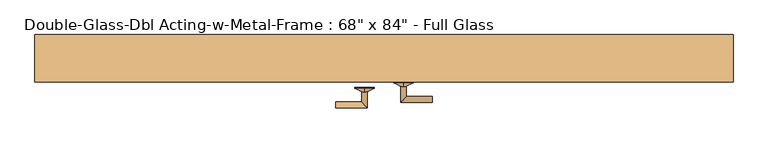
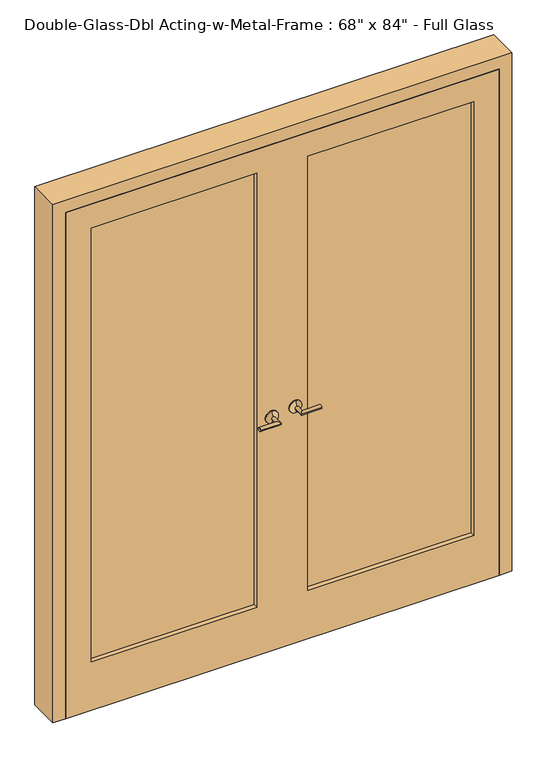
"""IFC4 building model written with IfcOpenShell, lengths in millimetres: door geometry."""

from ifc_helpers import new_model, si_unit, point, frame, origin, place, context, project, spatial, polyline, circle_curve, ellipse_curve, trimmed, outline, extrude, source, transform, mapped, element, save
from ifc_brep_helpers import plane_surface, cylinder_surface, revolved_surface, advanced_brep


def door_4d2e2016(model_context):
    return source(origin(), model_context, "Body", "SolidModel", [
        advanced_brep(
        [(50.8, -28.575, 971.55), (50.8, -28.575, 1022.35), (50.8, -20.0863821, 1004.45), (43.3, -20.0863821, 996.95), (50.8, -20.0863821, 989.45), (58.3, -20.0863821, 996.95), (50.8, -31.75, 971.55), (50.8, -31.75, 1022.35), (50.8, -31.75, 996.95), (43.3, 21.85, 996.95), (58.3, 6.85, 996.95), (125.8, 21.85, 996.95), (125.8, 6.85, 996.95)],
        [
            (0, 1, circle_curve(frame((50.8, -28.575, 996.95), z_axis=(0.0, 1.0, 0.0), x_axis=(0.0, 0.0, 1.0)), 25.4)),
            (1, 2, circle_curve(frame((50.8, 8.0292775, 1028.7458887), z_axis=(1.0000000000000004, 0.0, 0.0), x_axis=(0.0, 0.0, -1.0)), 37.1588553)),
            (2, 3, circle_curve(frame((50.8, -20.0863821, 996.95), z_axis=(0.0, -1.0, 0.0), x_axis=(0.0, 0.0, 1.0)), 7.5)),
            (3, 4, circle_curve(frame((50.8, -20.0863821, 996.95), z_axis=(0.0, -1.0, 0.0), x_axis=(0.0, 0.0, 1.0)), 7.5)),
            (4, 0, circle_curve(frame((50.8, 8.0292775, 965.1541113), z_axis=(1.0000000000000004, 0.0, 0.0), x_axis=(0.0, 0.0, 1.0)), 37.1588553)),
            (1, 0, circle_curve(frame((50.8, -28.575, 996.95), z_axis=(0.0, 1.0, 0.0), x_axis=(0.0, 0.0, 1.0)), 25.4)),
            (4, 5, circle_curve(frame((50.8, -20.0863821, 996.95), z_axis=(0.0, -1.0, 0.0), x_axis=(0.0, 0.0, 1.0)), 7.5)),
            (5, 2, circle_curve(frame((50.8, -20.0863821, 996.95), z_axis=(0.0, -1.0, 0.0), x_axis=(0.0, 0.0, 1.0)), 7.5)),
            (0, 6),
            (6, 7, circle_curve(frame((50.8, -31.75, 996.95), z_axis=(0.0, 1.0, 0.0), x_axis=(0.0, 0.0, 1.0)), 25.4)),
            (7, 1),
            (7, 6, circle_curve(frame((50.8, -31.75, 996.95), z_axis=(0.0, 1.0, 0.0), x_axis=(0.0, 0.0, 1.0)), 25.4)),
            (6, 8),
            (8, 7),
            (9, 10, ellipse_curve(frame((50.8, 14.35, 996.95), z_axis=(-0.7071067811864719, -0.7071067811866231, 0.0), x_axis=(0.707106781186623, -0.7071067811864721, 0.0)), 10.6066017, 7.5)),
            (10, 5),
            (3, 9),
            (10, 9, ellipse_curve(frame((50.8, 14.35, 996.95), z_axis=(-0.7071067811864719, -0.7071067811866231, 0.0), x_axis=(0.707106781186623, -0.7071067811864721, 0.0)), 10.6066017, 7.5)),
            (11, 12, circle_curve(frame((125.8, 14.35, 996.95), z_axis=(1.0, 0.0, 0.0), x_axis=(0.0, -1.0000000000000004, 0.0)), 7.5)),
            (12, 11, circle_curve(frame((125.8, 14.35, 996.95), z_axis=(1.0, 0.0, 0.0), x_axis=(0.0, -1.0000000000000004, 0.0)), 7.5)),
            (9, 11),
            (12, 10),
        ],
        [
            revolved_surface(trimmed(ellipse_curve(frame((50.8, 8.0292775, 1028.7458887), z_axis=(-1.0000000000000004, 0.0, 0.0), x_axis=(0.0, 0.0, -1.0)), 37.1588553, 37.1588553), [point((50.8, -19.05, 1003.3))], [point((50.8, -28.575, 1022.35))], True, "CARTESIAN"), (50.8, -19.05, 996.95), (0.0, -1.0000000000000004, 0.0)),
            cylinder_surface(frame((50.8, -19.05, 996.95), z_axis=(0.0, -1.0000000000000004, 0.0), x_axis=(0.0, 0.0, 1.0)), 25.4),
            plane_surface(frame((50.8, -31.75, 996.95), z_axis=(0.0, -1.0, 0.0), x_axis=(0.0, 0.0, 1.0))),
            cylinder_surface(frame((50.8, -23.75, 996.95), z_axis=(0.0, -1.0000000000000004, 0.0), x_axis=(1.0000000000000004, 0.0, 0.0)), 7.5),
            plane_surface(frame((125.8, 14.35, 996.95), z_axis=(1.0, 0.0, 0.0), x_axis=(0.0, 0.0, 1.0))),
            cylinder_surface(frame((50.8, 14.35, 996.95), z_axis=(-1.0000000000000004, 0.0, 0.0), x_axis=(0.0, -1.0000000000000004, 0.0)), 7.5),
        ],
        [
            (0, [[1, 2, 3, 4, 5]]),
            (0, [[6, -5, 7, 8, -2]]),
            (1, [[-1, 9, 10, 11]]),
            (1, [[-6, -11, 12, -9]]),
            (2, [[-10, 13, 14]]),
            (2, [[-12, -14, -13]]),
            (3, [[15, 16, -7, -4, 17]]),
            (3, [[18, -17, -3, -8, -16]]),
            (4, [[19, 20]]),
            (5, [[-15, 21, -20, 22]]),
            (5, [[-18, -22, -19, -21]]),
        ],
    ),
        advanced_brep(
        [(-50.8, -79.375, 971.55), (-50.8, -79.375, 1022.35), (-50.8, -87.8636179, 1004.45), (-43.3, -87.8636179, 996.95), (-50.8, -87.8636179, 989.45), (-58.3, -87.8636179, 996.95), (-50.8, -76.2, 971.55), (-50.8, -76.2, 1022.35), (-50.8, -76.2, 996.95), (-43.3, -129.8, 996.95), (-58.3, -114.8, 996.95), (-125.8, -129.8, 996.95), (-125.8, -114.8, 996.95)],
        [
            (0, 1, circle_curve(frame((-50.8, -79.375, 996.95), z_axis=(0.0, -1.0, 0.0), x_axis=(0.0, 0.0, 1.0)), 25.4)),
            (1, 2, circle_curve(frame((-50.8, -115.9792775, 1028.7458887), z_axis=(-1.0, 0.0, 0.0), x_axis=(0.0, 0.0, -1.0)), 37.1588553)),
            (2, 3, circle_curve(frame((-50.8, -87.8636179, 996.95), z_axis=(0.0, 1.0, 0.0), x_axis=(0.0, 0.0, 1.0)), 7.5)),
            (3, 4, circle_curve(frame((-50.8, -87.8636179, 996.95), z_axis=(0.0, 1.0, 0.0), x_axis=(0.0, 0.0, 1.0)), 7.5)),
            (4, 0, circle_curve(frame((-50.8, -115.9792775, 965.1541113), z_axis=(-1.0, 0.0, 0.0), x_axis=(0.0, 0.0, 1.0)), 37.1588553)),
            (1, 0, circle_curve(frame((-50.8, -79.375, 996.95), z_axis=(0.0, -1.0, 0.0), x_axis=(0.0, 0.0, 1.0)), 25.4)),
            (4, 5, circle_curve(frame((-50.8, -87.8636179, 996.95), z_axis=(0.0, 1.0, 0.0), x_axis=(0.0, 0.0, 1.0)), 7.5)),
            (5, 2, circle_curve(frame((-50.8, -87.8636179, 996.95), z_axis=(0.0, 1.0, 0.0), x_axis=(0.0, 0.0, 1.0)), 7.5)),
            (0, 6),
            (6, 7, circle_curve(frame((-50.8, -76.2, 996.95), z_axis=(0.0, -1.0, 0.0), x_axis=(0.0, 0.0, 1.0)), 25.4)),
            (7, 1),
            (7, 6, circle_curve(frame((-50.8, -76.2, 996.95), z_axis=(0.0, -1.0, 0.0), x_axis=(0.0, 0.0, 1.0)), 25.4)),
            (6, 8),
            (8, 7),
            (9, 10, ellipse_curve(frame((-50.8, -122.3, 996.95), z_axis=(0.7071067811864695, 0.7071067811866254, 0.0), x_axis=(-0.7071067811866254, 0.7071067811864696, 0.0)), 10.6066017, 7.5)),
            (10, 5),
            (3, 9),
            (10, 9, ellipse_curve(frame((-50.8, -122.3, 996.95), z_axis=(0.7071067811864695, 0.7071067811866254, 0.0), x_axis=(-0.7071067811866254, 0.7071067811864696, 0.0)), 10.6066017, 7.5)),
            (11, 12, circle_curve(frame((-125.8, -122.3, 996.95), z_axis=(-1.0, 0.0, 0.0), x_axis=(0.0, 1.0, 0.0)), 7.5)),
            (12, 11, circle_curve(frame((-125.8, -122.3, 996.95), z_axis=(-1.0, 0.0, 0.0), x_axis=(0.0, 1.0, 0.0)), 7.5)),
            (9, 11),
            (12, 10),
        ],
        [
            revolved_surface(trimmed(ellipse_curve(frame((-50.8, -115.9792775, 1028.7458887), z_axis=(1.0, 0.0, 0.0), x_axis=(0.0, 0.0, -1.0)), 37.1588553, 37.1588553), [point((-50.8, -88.9, 1003.3))], [point((-50.8, -79.375, 1022.35))], True, "CARTESIAN"), (-50.8, -88.9, 996.95), (0.0, 1.0, 0.0)),
            cylinder_surface(frame((-50.8, -88.9, 996.95), z_axis=(0.0, 1.0, 0.0), x_axis=(0.0, 0.0, 1.0)), 25.4),
            plane_surface(frame((-50.8, -76.2, 996.95), z_axis=(0.0, 1.0, 0.0), x_axis=(0.0, 0.0, 1.0))),
            cylinder_surface(frame((-50.8, -84.2, 996.95), z_axis=(0.0, 1.0, 0.0), x_axis=(-1.0, 0.0, 0.0)), 7.5),
            plane_surface(frame((-125.8, -122.3, 996.95), z_axis=(-1.0, 0.0, 0.0), x_axis=(0.0, 0.0, 1.0))),
            cylinder_surface(frame((-50.8, -122.3, 996.95), z_axis=(1.0, 0.0, 0.0), x_axis=(0.0, 1.0, 0.0)), 7.5),
        ],
        [
            (0, [[1, 2, 3, 4, 5]]),
            (0, [[6, -5, 7, 8, -2]]),
            (1, [[-1, 9, 10, 11]]),
            (1, [[-6, -11, 12, -9]]),
            (2, [[-10, 13, 14]]),
            (2, [[-12, -14, -13]]),
            (3, [[15, 16, -7, -4, 17]]),
            (3, [[18, -17, -3, -8, -16]]),
            (4, [[19, 20]]),
            (5, [[-15, 21, -20, 22]]),
            (5, [[-18, -22, -19, -21]]),
        ],
    ),
        advanced_brep(
        [(-50.8, -14.2875, 971.55), (-50.8, -5.7988821, 989.45), (-43.3, -5.7988821, 996.95), (-50.8, -5.7988821, 1004.45), (-50.8, -14.2875, 1022.35), (-58.3, -5.7988821, 996.95), (-50.8, -17.4625, 1022.35), (-50.8, -17.4625, 971.55), (-50.8, -17.4625, 996.95), (-43.3, 36.1375, 996.95), (-58.3, 21.1375, 996.95), (-125.8, 36.1375, 996.95), (-125.8, 21.1375, 996.95)],
        [
            (0, 1, circle_curve(frame((-50.8, 22.3167775, 965.1541113), z_axis=(-1.0, 0.0, 0.0), x_axis=(0.0, 0.0, 1.0)), 37.1588553)),
            (1, 2, circle_curve(frame((-50.8, -5.7988821, 996.95), z_axis=(0.0, -1.0, 0.0), x_axis=(0.0, 0.0, 1.0)), 7.5)),
            (2, 3, circle_curve(frame((-50.8, -5.7988821, 996.95), z_axis=(0.0, -1.0, 0.0), x_axis=(0.0, 0.0, 1.0)), 7.5)),
            (3, 4, circle_curve(frame((-50.8, 22.3167775, 1028.7458887), z_axis=(-1.0, 0.0, 0.0), x_axis=(0.0, 0.0, -1.0)), 37.1588553)),
            (4, 0, circle_curve(frame((-50.8, -14.2875, 996.95), z_axis=(0.0, 1.0, 0.0), x_axis=(0.0, 0.0, 1.0)), 25.4)),
            (3, 5, circle_curve(frame((-50.8, -5.7988821, 996.95), z_axis=(0.0, -1.0, 0.0), x_axis=(0.0, 0.0, 1.0)), 7.5)),
            (5, 1, circle_curve(frame((-50.8, -5.7988821, 996.95), z_axis=(0.0, -1.0, 0.0), x_axis=(0.0, 0.0, 1.0)), 7.5)),
            (0, 4, circle_curve(frame((-50.8, -14.2875, 996.95), z_axis=(0.0, 1.0, 0.0), x_axis=(0.0, 0.0, 1.0)), 25.4)),
            (4, 6),
            (6, 7, circle_curve(frame((-50.8, -17.4625, 996.95), z_axis=(0.0, 1.0, 0.0), x_axis=(0.0, 0.0, 1.0)), 25.4)),
            (7, 0),
            (7, 6, circle_curve(frame((-50.8, -17.4625, 996.95), z_axis=(0.0, 1.0, 0.0), x_axis=(0.0, 0.0, 1.0)), 25.4)),
            (6, 8),
            (8, 7),
            (9, 2),
            (5, 10),
            (10, 9, ellipse_curve(frame((-50.8, 28.6375, 996.95), z_axis=(0.7071067811864719, -0.7071067811866231, 0.0), x_axis=(-0.707106781186623, -0.7071067811864721, 0.0)), 10.6066017, 7.5)),
            (9, 10, ellipse_curve(frame((-50.8, 28.6375, 996.95), z_axis=(0.7071067811864719, -0.7071067811866231, 0.0), x_axis=(-0.707106781186623, -0.7071067811864721, 0.0)), 10.6066017, 7.5)),
            (11, 12, circle_curve(frame((-125.8, 28.6375, 996.95), z_axis=(-1.0, 0.0, 0.0), x_axis=(0.0, -1.0, 0.0)), 7.5)),
            (12, 11, circle_curve(frame((-125.8, 28.6375, 996.95), z_axis=(-1.0, 0.0, 0.0), x_axis=(0.0, -1.0, 0.0)), 7.5)),
            (10, 12),
            (11, 9),
        ],
        [
            revolved_surface(trimmed(ellipse_curve(frame((-50.8, 22.3167775, 1028.7458887), z_axis=(-1.0, 0.0, 0.0), x_axis=(0.0, 0.0, -1.0)), 37.1588553, 37.1588553), [point((-50.8, -4.7625, 1003.3))], [point((-50.8, -14.2875, 1022.35))], True, "CARTESIAN"), (-50.8, -4.7625, 996.95), (0.0, -1.0, 0.0)),
            cylinder_surface(frame((-50.8, -4.7625, 996.95), z_axis=(0.0, -1.0, 0.0), x_axis=(0.0, 0.0, 1.0)), 25.4),
            plane_surface(frame((-50.8, -17.4625, 996.95), z_axis=(0.0, -1.0, 0.0), x_axis=(0.0, 0.0, 1.0))),
            cylinder_surface(frame((-50.8, -9.4625, 996.95), z_axis=(0.0, -1.0, 0.0), x_axis=(-1.0, 0.0, 0.0)), 7.5),
            plane_surface(frame((-125.8, 28.6375, 996.95), z_axis=(-1.0, 0.0, 0.0), x_axis=(0.0, 0.0, 1.0))),
            cylinder_surface(frame((-50.8, 28.6375, 996.95), z_axis=(1.0, 0.0, 0.0), x_axis=(0.0, -1.0, 0.0)), 7.5),
        ],
        [
            (0, [[1, 2, 3, 4, 5]]),
            (0, [[-4, 6, 7, -1, 8]]),
            (1, [[9, 10, 11, -5]]),
            (1, [[-11, 12, -9, -8]]),
            (2, [[13, 14, -10]]),
            (2, [[-14, -13, -12]]),
            (3, [[15, -2, -7, 16, 17]]),
            (3, [[-16, -6, -3, -15, 18]]),
            (4, [[19, 20]]),
            (5, [[21, -19, 22, -17]]),
            (5, [[-22, -20, -21, -18]]),
        ],
    ),
        advanced_brep(
        [(50.8, -65.0875, 971.55), (50.8, -73.5761179, 989.45), (43.3, -73.5761179, 996.95), (50.8, -73.5761179, 1004.45), (50.8, -65.0875, 1022.35), (58.3, -73.5761179, 996.95), (50.8, -61.9125, 1022.35), (50.8, -61.9125, 971.55), (50.8, -61.9125, 996.95), (43.3, -115.5125, 996.95), (58.3, -100.5125, 996.95), (125.8, -115.5125, 996.95), (125.8, -100.5125, 996.95)],
        [
            (0, 1, circle_curve(frame((50.8, -101.6917775, 965.1541113), z_axis=(1.0, 0.0, 0.0), x_axis=(0.0, 0.0, 1.0)), 37.1588553)),
            (1, 2, circle_curve(frame((50.8, -73.5761179, 996.95), z_axis=(0.0, 1.0, 0.0), x_axis=(0.0, 0.0, 1.0)), 7.5)),
            (2, 3, circle_curve(frame((50.8, -73.5761179, 996.95), z_axis=(0.0, 1.0, 0.0), x_axis=(0.0, 0.0, 1.0)), 7.5)),
            (3, 4, circle_curve(frame((50.8, -101.6917775, 1028.7458887), z_axis=(1.0, 0.0, 0.0), x_axis=(0.0, 0.0, -1.0)), 37.1588553)),
            (4, 0, circle_curve(frame((50.8, -65.0875, 996.95), z_axis=(0.0, -1.0, 0.0), x_axis=(0.0, 0.0, 1.0)), 25.4)),
            (3, 5, circle_curve(frame((50.8, -73.5761179, 996.95), z_axis=(0.0, 1.0, 0.0), x_axis=(0.0, 0.0, 1.0)), 7.5)),
            (5, 1, circle_curve(frame((50.8, -73.5761179, 996.95), z_axis=(0.0, 1.0, 0.0), x_axis=(0.0, 0.0, 1.0)), 7.5)),
            (0, 4, circle_curve(frame((50.8, -65.0875, 996.95), z_axis=(0.0, -1.0, 0.0), x_axis=(0.0, 0.0, 1.0)), 25.4)),
            (4, 6),
            (6, 7, circle_curve(frame((50.8, -61.9125, 996.95), z_axis=(0.0, -1.0, 0.0), x_axis=(0.0, 0.0, 1.0)), 25.4)),
            (7, 0),
            (7, 6, circle_curve(frame((50.8, -61.9125, 996.95), z_axis=(0.0, -1.0, 0.0), x_axis=(0.0, 0.0, 1.0)), 25.4)),
            (6, 8),
            (8, 7),
            (9, 2),
            (5, 10),
            (10, 9, ellipse_curve(frame((50.8, -108.0125, 996.95), z_axis=(-0.7071067811864695, 0.7071067811866254, 0.0), x_axis=(0.7071067811866254, 0.7071067811864696, 0.0)), 10.6066017, 7.5)),
            (9, 10, ellipse_curve(frame((50.8, -108.0125, 996.95), z_axis=(-0.7071067811864695, 0.7071067811866254, 0.0), x_axis=(0.7071067811866254, 0.7071067811864696, 0.0)), 10.6066017, 7.5)),
            (11, 12, circle_curve(frame((125.8, -108.0125, 996.95), z_axis=(1.0, 0.0, 0.0), x_axis=(0.0, 1.0, 0.0)), 7.5)),
            (12, 11, circle_curve(frame((125.8, -108.0125, 996.95), z_axis=(1.0, 0.0, 0.0), x_axis=(0.0, 1.0, 0.0)), 7.5)),
            (10, 12),
            (11, 9),
        ],
        [
            revolved_surface(trimmed(ellipse_curve(frame((50.8, -101.6917775, 1028.7458887), z_axis=(1.0, 0.0, 0.0), x_axis=(0.0, 0.0, -1.0)), 37.1588553, 37.1588553), [point((50.8, -74.6125, 1003.3))], [point((50.8, -65.0875, 1022.35))], True, "CARTESIAN"), (50.8, -74.6125, 996.95), (0.0, 1.0, 0.0)),
            cylinder_surface(frame((50.8, -74.6125, 996.95), z_axis=(0.0, 1.0, 0.0), x_axis=(0.0, 0.0, 1.0)), 25.4),
            plane_surface(frame((50.8, -61.9125, 996.95), z_axis=(0.0, 1.0, 0.0), x_axis=(0.0, 0.0, 1.0))),
            cylinder_surface(frame((50.8, -69.9125, 996.95), z_axis=(0.0, 1.0, 0.0), x_axis=(1.0, 0.0, 0.0)), 7.5),
            plane_surface(frame((125.8, -108.0125, 996.95), z_axis=(1.0, 0.0, 0.0), x_axis=(0.0, 0.0, 1.0))),
            cylinder_surface(frame((50.8, -108.0125, 996.95), z_axis=(-1.0, 0.0, 0.0), x_axis=(0.0, 1.0, 0.0)), 7.5),
        ],
        [
            (0, [[1, 2, 3, 4, 5]]),
            (0, [[-4, 6, 7, -1, 8]]),
            (1, [[9, 10, 11, -5]]),
            (1, [[-11, 12, -9, -8]]),
            (2, [[13, 14, -10]]),
            (2, [[-14, -13, -12]]),
            (3, [[15, -2, -7, 16, 17]]),
            (3, [[-16, -6, -3, -15, 18]]),
            (4, [[19, 20]]),
            (5, [[21, -19, 22, -17]]),
            (5, [[-22, -20, -21, -18]]),
        ],
    ),
        extrude(outline(polyline([(-762.0, -42.8625), (-762.0, -36.5125), (-101.6, -36.5125), (-101.6, -42.8625), (-762.0, -42.8625)])), frame((0.0, 0.0, 203.2), z_axis=(0.0, 0.0, 1.0), x_axis=(1.0, 0.0, 0.0)), (0.0, 0.0, 1.0), 1828.8),
        extrude(outline(polyline([(101.6, -42.8625), (101.6, -36.5125), (762.0, -36.5125), (762.0, -42.8625), (101.6, -42.8625)])), frame((0.0, 0.0, 203.2), z_axis=(0.0, 0.0, 1.0), x_axis=(1.0, 0.0, 0.0)), (0.0, 0.0, 1.0), 1828.8),
        extrude(outline(polyline([(2133.6, -863.6), (0.0, -863.6), (0.0, 863.6), (2133.6, 863.6), (2133.6, -863.6)]), holes=[polyline([(2032.0, -101.6), (203.2, -101.6), (203.2, -762.0), (2032.0, -762.0), (2032.0, -101.6)]), polyline([(2032.0, 762.0), (203.2, 762.0), (203.2, 101.6), (2032.0, 101.6), (2032.0, 762.0)])]), frame((0.0, -61.9125, 0.0), z_axis=(0.0, 1.0, 0.0), x_axis=(0.0, 0.0, 1.0)), (0.0, 0.0, 1.0), 44.45),
        extrude(outline(polyline([(0.0, -863.6), (2133.6, -863.6), (2133.6, 863.6), (0.0, 863.6), (0.0, 914.4), (2184.4, 914.4), (2184.4, -914.4), (0.0, -914.4), (0.0, -863.6)])), frame((0.0, -61.9125, 0.0), z_axis=(0.0, 1.0, 0.0), x_axis=(0.0, 0.0, 1.0)), (0.0, 0.0, 1.0), 123.825),
    ])


if __name__ == "__main__":
    model = new_model("IFC4")
    model_context = context("Model", 3, world=origin())
    ifc_project = project(units=[si_unit("LENGTHUNIT", "METRE", prefix="MILLI")], contexts=[model_context])
    site = spatial("IfcSite", under=ifc_project)
    building = spatial("IfcBuilding", under=site)
    placement = place(None, origin())
    door_shape = door_4d2e2016(model_context)
    element("IfcDoor", 1, ObjectType="Double-Glass-Dbl Acting-w-Metal-Frame : 68\" x 84\" - Full Glass", at=placement, inside=building, context=model_context, shape_type="MappedRepresentation", body=[
        mapped(door_shape, transform((0.0, 0.0, 0.0), x_axis=(1.0, 0.0, 0.0), y_axis=(0.0, 1.0, 0.0), z_axis=(0.0, 0.0, 1.0))),
    ])
    save(model, "model.ifc")

# Revit data of these elements
# Type "Double-Glass-Dbl Acting-w-Metal-Frame : 68\" x 84\" - Full Glass"
#   Type Mark = "11"
#   Construction Type Id = "MDOOR"
#   Assembly Code = "C1020"
#   Analytic Construction = "Metal"
#   Top Rail = 0' - 4"
#   Thickness = 0' - 1 3/4"
#   Thermal Resistance (R) = 1.5338 (h·ft²·°F)/BTU
#   Rough Width = 5' - 10"
#   Rough Height = 7' - 2"
#   Right Side Rail = 0' - 4"
#   Left Side Rail = 0' - 4"
#   Half Width Neg = -3' - 0"
#   Half Width = 3' - 0"
#   Frame Width = 0' - 2"
#   Frame Head Height = 0' - 2"
#   Heat Transfer Coefficient (U) = 0.651978 BTU/(h·ft²·°F)
#   Bottom Rail = 0' - 8"
#   Height = 7' - 0"
#   Width = 5' - 8"
#   Define Thermal Properties by = 1
#   Define Thermal Properties by = 1
#   Door Material = Aluminum Painted - Red
#   Frame Material = Aluminum Painted - Red
#   Visual Light Transmittance = 0
#   Solar Heat Gain Coefficient = 0
#   Function = (empty or 0)
#   Wall Closure = (empty or 0)
# Element 1 (IfcDoor, "Double-Glass-Dbl Acting-w-Metal-Frame : 68\" x 84\" - Full Glass")
#   Materials on its faces: "Metal - Aluminium", "Aluminum Painted - Red", "Glass"
# Materials
#   "Aluminum Painted - Red": class "Metal", colour RGB 255 0 0, transparency 0, Description = "Aluminum 6061", Cost = 0
#   "Metal - Aluminium": class "Unassigned", colour RGB 247 247 247, transparency 0
#   "Glass": class "Glass", colour RGB 0 128 192, transparency 0.75, Description = "Soda Lime Glass", Cost = 0
